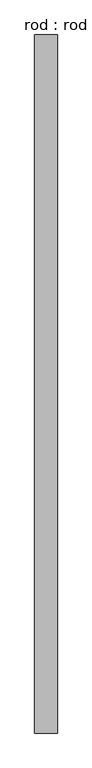
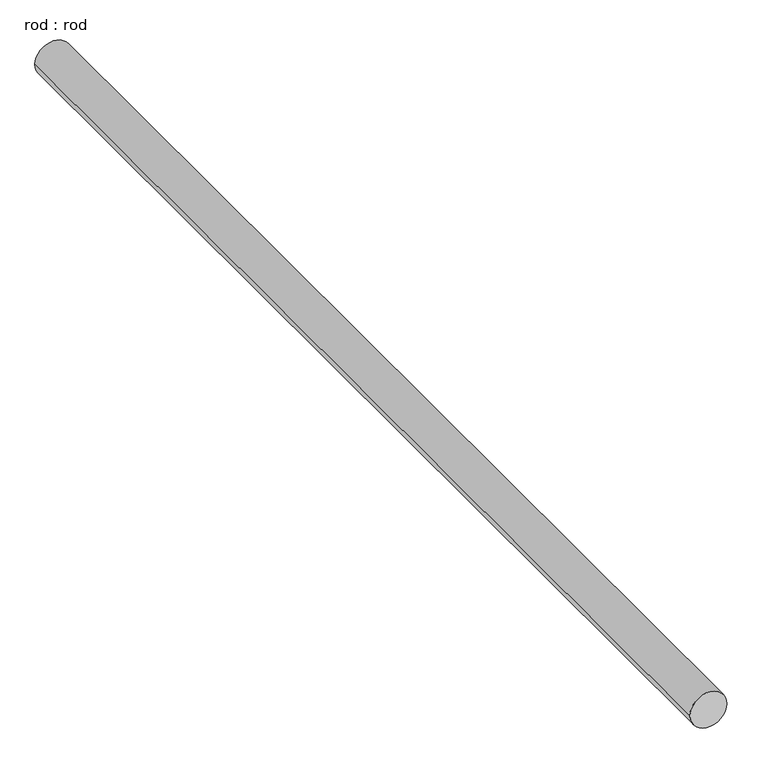
"""IFC4 building model written with IfcOpenShell, lengths in millimetres: proxy geometry, rod : rod."""

from ifc_helpers import new_model, si_unit, point, frame, frame_2d, origin, place, context, project, spatial, circle_curve, trimmed, segment, composite_curve, outline, extrude, source, transform, mapped, element, save


def rod_rod_12c3e847(model_context):
    return source(origin(), model_context, "Body", "SweptSolid", [
        extrude(outline(composite_curve([segment(trimmed(circle_curve(frame_2d((0.0108462, 0.0)), 200.0), [point((0.0108462, 200.0))], [point((0.0108462, -200.0))], False, "CARTESIAN"), True, "CONTINUOUS"), segment(trimmed(circle_curve(frame_2d((0.0108462, 0.0)), 200.0), [point((0.0108462, -200.0))], [point((0.0108462, 200.0))], False, "CARTESIAN"), True, "CONTINUOUS")], self_intersect=False)), frame((0.0, -2088.1615129, 0.0), z_axis=(0.0, 1.0, 0.0), x_axis=(0.0, 0.0, 1.0)), (0.0, 0.0, 1.0), 12361.7802565),
    ])


if __name__ == "__main__":
    model = new_model("IFC4")
    model_context = context("Model", 3, world=origin())
    ifc_project = project(units=[si_unit("LENGTHUNIT", "METRE", prefix="MILLI")], contexts=[model_context])
    site = spatial("IfcSite", under=ifc_project)
    building = spatial("IfcBuilding", under=site)
    placement = place(None, origin())
    rod_rod_shape = rod_rod_12c3e847(model_context)
    element("IfcBuildingElementProxy", 1, Name="rod : rod", ObjectType="rod : rod", at=placement, inside=building, context=model_context, shape_type="MappedRepresentation", body=[
        mapped(rod_rod_shape, transform((0.0, 0.0, 0.0), x_axis=(1.0, 0.0, 0.0), y_axis=(0.0, 1.0, 0.0), z_axis=(0.0, 0.0, 1.0))),
    ])
    save(model, "model.ifc")

# Revit data of these elements
# Type "rod : rod"
#   Default Elevation = 0
